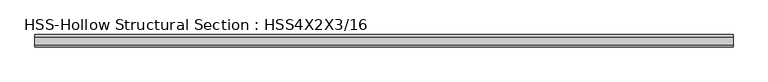
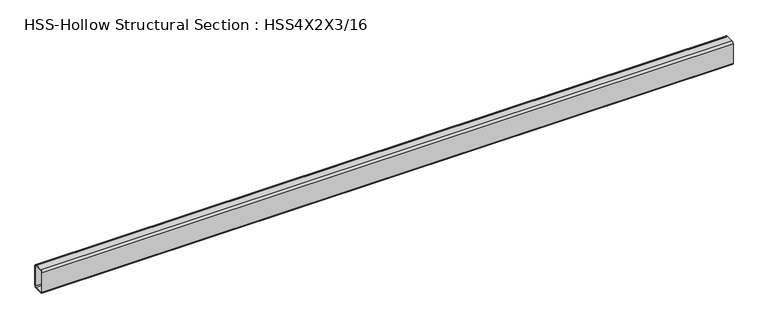
"""IFC4 building model written with IfcOpenShell, lengths in millimetres: beam geometry, HSS-Hollow Structural Section : HSS4X2X3/16."""

from ifc_helpers import new_model, si_unit, point, frame, frame_2d, origin, place, context, project, spatial, polyline, circle_curve, trimmed, segment, composite_curve, outline, extrude, source, transform, mapped, element, save


def hss_hollow_structural_section_hss4x2x3_16_c92bde9d(model_context):
    return source(origin(), model_context, "Body", "SweptSolid", [
        extrude(outline(composite_curve([segment(polyline([(25.4, 41.9608), (25.4, -41.9608)]), True, "CONTINUOUS"), segment(trimmed(circle_curve(frame_2d((16.5608, -41.9608)), 8.8392), [point((25.4, -41.9608))], [point((16.5608, -50.8))], False, "CARTESIAN"), True, "CONTINUOUS"), segment(polyline([(16.5608, -50.8), (-16.5608, -50.8)]), True, "CONTINUOUS"), segment(trimmed(circle_curve(frame_2d((-16.5608, -41.9608)), 8.8392), [point((-16.5608, -50.8))], [point((-25.4, -41.9608))], False, "CARTESIAN"), True, "CONTINUOUS"), segment(polyline([(-25.4, -41.9608), (-25.4, 41.9608)]), True, "CONTINUOUS"), segment(trimmed(circle_curve(frame_2d((-16.5608, 41.9608)), 8.8392), [point((-25.4, 41.9608))], [point((-16.5608, 50.8))], False, "CARTESIAN"), True, "CONTINUOUS"), segment(polyline([(-16.5608, 50.8), (16.5608, 50.8)]), True, "CONTINUOUS"), segment(trimmed(circle_curve(frame_2d((16.5608, 41.9608)), 8.8392), [point((16.5608, 50.8))], [point((25.4, 41.9608))], False, "CARTESIAN"), True, "CONTINUOUS")], self_intersect=False), holes=[composite_curve([segment(trimmed(circle_curve(frame_2d((-16.5608, 41.9608)), 4.4196), [point((-16.5608, 46.3804))], [point((-20.9804, 41.9608))], True, "CARTESIAN"), True, "CONTINUOUS"), segment(polyline([(-20.9804, 41.9608), (-20.9804, -41.9608)]), True, "CONTINUOUS"), segment(trimmed(circle_curve(frame_2d((-16.5608, -41.9608)), 4.4196), [point((-20.9804, -41.9608))], [point((-16.5608, -46.3804))], True, "CARTESIAN"), True, "CONTINUOUS"), segment(polyline([(-16.5608, -46.3804), (16.5608, -46.3804)]), True, "CONTINUOUS"), segment(trimmed(circle_curve(frame_2d((16.5608, -41.9608)), 4.4196), [point((16.5608, -46.3804))], [point((20.9804, -41.9608))], True, "CARTESIAN"), True, "CONTINUOUS"), segment(polyline([(20.9804, -41.9608), (20.9804, 41.9608)]), True, "CONTINUOUS"), segment(trimmed(circle_curve(frame_2d((16.5608, 41.9608)), 4.4196), [point((20.9804, 41.9608))], [point((16.5608, 46.3804))], True, "CARTESIAN"), True, "CONTINUOUS"), segment(polyline([(16.5608, 46.3804), (-16.5608, 46.3804)]), True, "CONTINUOUS")], self_intersect=False)]), frame((-533.4, 0.0, 0.0), z_axis=(1.0, 0.0, 0.0), x_axis=(0.0, 1.0, 0.0)), (0.0, 0.0, 1.0), 2860.0936767),
    ])


if __name__ == "__main__":
    model = new_model("IFC4")
    model_context = context("Model", 3, world=origin())
    ifc_project = project(units=[si_unit("LENGTHUNIT", "METRE", prefix="MILLI")], contexts=[model_context])
    site = spatial("IfcSite", under=ifc_project)
    building = spatial("IfcBuilding", under=site)
    placement = place(None, origin())
    hss_hollow_structural_section_hss4x2x3_16_shape = hss_hollow_structural_section_hss4x2x3_16_c92bde9d(model_context)
    element("IfcBeam", 1, ObjectType="HSS-Hollow Structural Section : HSS4X2X3/16", at=placement, inside=building, context=model_context, shape_type="MappedRepresentation", body=[
        mapped(hss_hollow_structural_section_hss4x2x3_16_shape, transform((0.0, 0.0, 0.0), x_axis=(1.0, 0.0, 0.0), y_axis=(0.0, 1.0, 0.0), z_axis=(0.0, 0.0, 1.0))),
    ])
    save(model, "model.ifc")

# Revit data of these elements
# Type "HSS-Hollow Structural Section : HSS4X2X3/16"
#   Assembly Code = "B10"
#   Shape = "Rect."
#   W = 6.87
#   Ht = 0' - 4"
#   Length [instance default] = 5' - 0"
#   b = 0' - 2"
#   kr = 0' - 0.348"
#   t = 0' - 0.174"
#   A = 0.013125 SF
#   Structural Material [instance default] = none
# Element 1 (IfcBeam, "HSS-Hollow Structural Section : HSS4X2X3/16")
#   Structural Material = _2x3 STEEL PROFILE - METALIZED, PRIMED & PAINTED (COLOR PER ARCHITECT)
#   Materials on its faces: "_2x3 STEEL PROFILE - METALIZED, PRIMED & PAINTED (COLOR PER ARCHITECT)"
# Materials
#   "_2x3 STEEL PROFILE - METALIZED, PRIMED & PAINTED (COLOR PER ARCHITECT)": class "Metal", colour RGB 199 199 199, transparency 0, Description = "Structural steel 50ksi", Cost = 0
